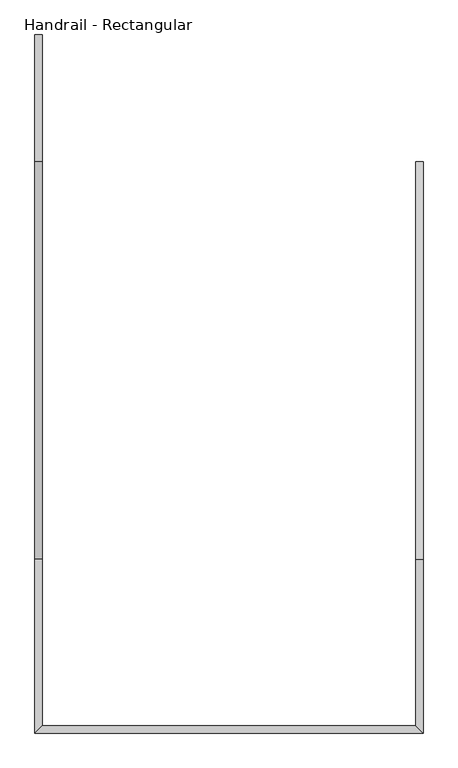
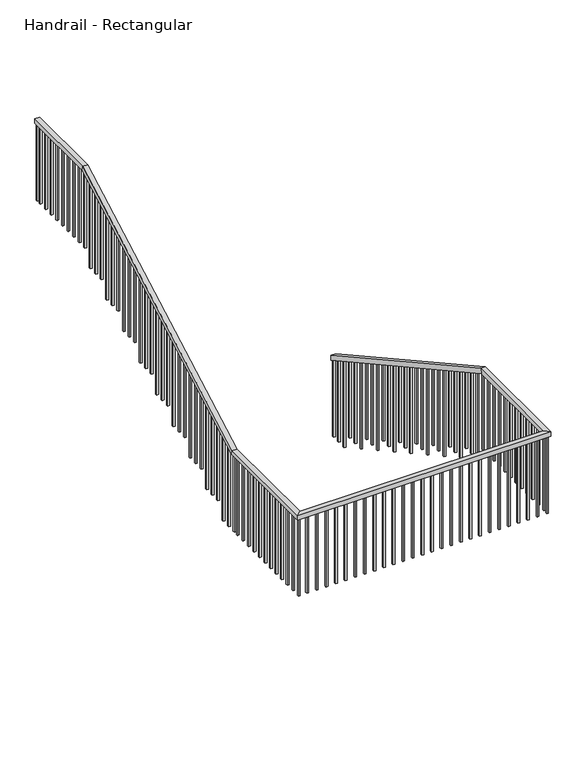
"""IFC4 building model written with IfcOpenShell, lengths in millimetres: railing geometry, Handrail - Rectangular."""

from ifc_helpers import new_model, si_unit, frame, origin, place, context, project, spatial, polyline, outline, extrude, faceted_brep, source, transform, mapped, element, save


def handrail_rectangular_0e0fe6d2(model_context):
    return source(origin(), model_context, "Body", "SolidModel", [
        faceted_brep([(-73320.227375, 12915.9, 10449.0921053), (-73269.427375, 12915.9, 10449.0921053), (-73269.427375, 12915.9, 10391.0509841), (-73320.227375, 12915.9, 10391.0509841), (-73320.227375, 10172.7, 11965.0710526), (-73269.427375, 10172.7, 11965.0710526), (-73269.427375, 10159.5970189, 11914.2710526), (-73320.227375, 10159.5970189, 11914.2710526), (-73320.227375, 9023.35, 11965.0710526), (-73269.427375, 8972.55, 11965.0710526), (-73269.427375, 8972.55, 11914.2710526), (-73320.227375, 9023.35, 11914.2710526), (-75898.327375, 9023.35, 11965.0710526), (-75949.127375, 8972.55, 11965.0710526), (-75949.127375, 8972.55, 11914.2710526), (-75898.327375, 9023.35, 11914.2710526), (-75898.327375, 10172.7, 11965.0710526), (-75949.127375, 10172.7, 11965.0710526), (-75949.127375, 10185.8029811, 11914.2710526), (-75898.327375, 10185.8029811, 11914.2710526), (-75898.327375, 12915.9, 13481.05), (-75949.127375, 12915.9, 13481.05), (-75949.127375, 12929.0029811, 13430.25), (-75898.327375, 12929.0029811, 13430.25), (-75898.327375, 13792.2, 13481.05), (-75898.327375, 13792.2, 13430.25), (-75949.127375, 13792.2, 13430.25), (-75949.127375, 13792.2, 13481.05)], [[[0, 1, 2, 3]], [[1, 0, 4, 5]], [[2, 1, 5, 6]], [[3, 2, 6, 7]], [[0, 3, 7, 4]], [[5, 4, 8, 9]], [[6, 5, 9, 10]], [[7, 6, 10, 11]], [[4, 7, 11, 8]], [[9, 8, 12, 13]], [[10, 9, 13, 14]], [[11, 10, 14, 15]], [[8, 11, 15, 12]], [[13, 12, 16, 17]], [[14, 13, 17, 18]], [[15, 14, 18, 19]], [[12, 15, 19, 16]], [[17, 16, 20, 21]], [[18, 17, 21, 22]], [[19, 18, 22, 23]], [[16, 19, 23, 20]], [[24, 25, 26, 27]], [[21, 20, 24, 27]], [[22, 21, 27, 26]], [[23, 22, 26, 25]], [[20, 23, 25, 24]]]),
        extrude(outline(polyline([(-75914.202375, 13719.175), (-75933.252375, 13719.175), (-75933.252375, 13738.225), (-75914.202375, 13738.225), (-75914.202375, 13719.175)])), frame((0.0, 0.0, 12566.65), z_axis=(0.0, 0.0, 1.0), x_axis=(1.0, 0.0, 0.0)), (0.0, 0.0, 1.0), 863.6),
        extrude(outline(polyline([(-75914.202375, 13617.575), (-75933.252375, 13617.575), (-75933.252375, 13636.625), (-75914.202375, 13636.625), (-75914.202375, 13617.575)])), frame((0.0, 0.0, 12566.65), z_axis=(0.0, 0.0, 1.0), x_axis=(1.0, 0.0, 0.0)), (0.0, 0.0, 1.0), 863.6),
        extrude(outline(polyline([(-75914.202375, 13515.975), (-75933.252375, 13515.975), (-75933.252375, 13535.025), (-75914.202375, 13535.025), (-75914.202375, 13515.975)])), frame((0.0, 0.0, 12566.65), z_axis=(0.0, 0.0, 1.0), x_axis=(1.0, 0.0, 0.0)), (0.0, 0.0, 1.0), 863.6),
        extrude(outline(polyline([(-75914.202375, 13414.375), (-75933.252375, 13414.375), (-75933.252375, 13433.425), (-75914.202375, 13433.425), (-75914.202375, 13414.375)])), frame((0.0, 0.0, 12566.65), z_axis=(0.0, 0.0, 1.0), x_axis=(1.0, 0.0, 0.0)), (0.0, 0.0, 1.0), 863.6),
        extrude(outline(polyline([(-75914.202375, 13312.775), (-75933.252375, 13312.775), (-75933.252375, 13331.825), (-75914.202375, 13331.825), (-75914.202375, 13312.775)])), frame((0.0, 0.0, 12566.65), z_axis=(0.0, 0.0, 1.0), x_axis=(1.0, 0.0, 0.0)), (0.0, 0.0, 1.0), 863.6),
        extrude(outline(polyline([(-75914.202375, 13211.175), (-75933.252375, 13211.175), (-75933.252375, 13230.225), (-75914.202375, 13230.225), (-75914.202375, 13211.175)])), frame((0.0, 0.0, 12566.65), z_axis=(0.0, 0.0, 1.0), x_axis=(1.0, 0.0, 0.0)), (0.0, 0.0, 1.0), 863.6),
        extrude(outline(polyline([(-75914.202375, 13109.575), (-75933.252375, 13109.575), (-75933.252375, 13128.625), (-75914.202375, 13128.625), (-75914.202375, 13109.575)])), frame((0.0, 0.0, 12566.65), z_axis=(0.0, 0.0, 1.0), x_axis=(1.0, 0.0, 0.0)), (0.0, 0.0, 1.0), 863.6),
        extrude(outline(polyline([(-75914.202375, 13007.975), (-75933.252375, 13007.975), (-75933.252375, 13027.025), (-75914.202375, 13027.025), (-75914.202375, 13007.975)])), frame((0.0, 0.0, 12566.65), z_axis=(0.0, 0.0, 1.0), x_axis=(1.0, 0.0, 0.0)), (0.0, 0.0, 1.0), 863.6),
        extrude(outline(polyline([(12804.775, 13361.5976946), (12823.825, 13372.1253262), (12823.825, 12398.2078947), (12804.775, 12398.2078947), (12804.775, 13361.5976946)])), frame((-75933.252375, 0.0, 0.0), z_axis=(1.0, 0.0, 0.0), x_axis=(0.0, 1.0, 0.0)), (0.0, 0.0, 1.0), 19.05),
        extrude(outline(polyline([(12703.175, 13305.4503262), (12722.225, 13315.9779578), (12722.225, 12398.2078947), (12703.175, 12398.2078947), (12703.175, 13305.4503262)])), frame((-75933.252375, 0.0, 0.0), z_axis=(1.0, 0.0, 0.0), x_axis=(0.0, 1.0, 0.0)), (0.0, 0.0, 1.0), 19.05),
        extrude(outline(polyline([(12601.575, 13249.3029578), (12620.625, 13259.8305894), (12620.625, 12398.2078947), (12601.575, 12398.2078947), (12601.575, 13249.3029578)])), frame((-75933.252375, 0.0, 0.0), z_axis=(1.0, 0.0, 0.0), x_axis=(0.0, 1.0, 0.0)), (0.0, 0.0, 1.0), 19.05),
        extrude(outline(polyline([(12499.975, 13193.1555894), (12519.025, 13203.6832209), (12519.025, 12229.7657895), (12499.975, 12229.7657895), (12499.975, 13193.1555894)])), frame((-75933.252375, 0.0, 0.0), z_axis=(1.0, 0.0, 0.0), x_axis=(0.0, 1.0, 0.0)), (0.0, 0.0, 1.0), 19.05),
        extrude(outline(polyline([(12398.375, 13137.0082209), (12417.425, 13147.5358525), (12417.425, 12229.7657895), (12398.375, 12229.7657895), (12398.375, 13137.0082209)])), frame((-75933.252375, 0.0, 0.0), z_axis=(1.0, 0.0, 0.0), x_axis=(0.0, 1.0, 0.0)), (0.0, 0.0, 1.0), 19.05),
        extrude(outline(polyline([(12296.775, 13080.8608525), (12315.825, 13091.3884841), (12315.825, 12229.7657895), (12296.775, 12229.7657895), (12296.775, 13080.8608525)])), frame((-75933.252375, 0.0, 0.0), z_axis=(1.0, 0.0, 0.0), x_axis=(0.0, 1.0, 0.0)), (0.0, 0.0, 1.0), 19.05),
        extrude(outline(polyline([(12195.175, 13024.7134841), (12214.225, 13035.2411157), (12214.225, 12061.3236842), (12195.175, 12061.3236842), (12195.175, 13024.7134841)])), frame((-75933.252375, 0.0, 0.0), z_axis=(1.0, 0.0, 0.0), x_axis=(0.0, 1.0, 0.0)), (0.0, 0.0, 1.0), 19.05),
        extrude(outline(polyline([(12093.575, 12968.5661157), (12112.625, 12979.0937473), (12112.625, 12061.3236842), (12093.575, 12061.3236842), (12093.575, 12968.5661157)])), frame((-75933.252375, 0.0, 0.0), z_axis=(1.0, 0.0, 0.0), x_axis=(0.0, 1.0, 0.0)), (0.0, 0.0, 1.0), 19.05),
        extrude(outline(polyline([(11991.975, 12912.4187473), (12011.025, 12922.9463788), (12011.025, 12061.3236842), (11991.975, 12061.3236842), (11991.975, 12912.4187473)])), frame((-75933.252375, 0.0, 0.0), z_axis=(1.0, 0.0, 0.0), x_axis=(0.0, 1.0, 0.0)), (0.0, 0.0, 1.0), 19.05),
        extrude(outline(polyline([(11890.375, 12856.2713788), (11909.425, 12866.7990104), (11909.425, 11892.8815789), (11890.375, 11892.8815789), (11890.375, 12856.2713788)])), frame((-75933.252375, 0.0, 0.0), z_axis=(1.0, 0.0, 0.0), x_axis=(0.0, 1.0, 0.0)), (0.0, 0.0, 1.0), 19.05),
        extrude(outline(polyline([(11788.775, 12800.1240104), (11807.825, 12810.651642), (11807.825, 11892.8815789), (11788.775, 11892.8815789), (11788.775, 12800.1240104)])), frame((-75933.252375, 0.0, 0.0), z_axis=(1.0, 0.0, 0.0), x_axis=(0.0, 1.0, 0.0)), (0.0, 0.0, 1.0), 19.05),
        extrude(outline(polyline([(11687.175, 12743.976642), (11706.225, 12754.5042736), (11706.225, 11892.8815789), (11687.175, 11892.8815789), (11687.175, 12743.976642)])), frame((-75933.252375, 0.0, 0.0), z_axis=(1.0, 0.0, 0.0), x_axis=(0.0, 1.0, 0.0)), (0.0, 0.0, 1.0), 19.05),
        extrude(outline(polyline([(11585.575, 12687.8292736), (11604.625, 12698.3569052), (11604.625, 11724.4394737), (11585.575, 11724.4394737), (11585.575, 12687.8292736)])), frame((-75933.252375, 0.0, 0.0), z_axis=(1.0, 0.0, 0.0), x_axis=(0.0, 1.0, 0.0)), (0.0, 0.0, 1.0), 19.05),
        extrude(outline(polyline([(11483.975, 12631.6819052), (11503.025, 12642.2095367), (11503.025, 11724.4394737), (11483.975, 11724.4394737), (11483.975, 12631.6819052)])), frame((-75933.252375, 0.0, 0.0), z_axis=(1.0, 0.0, 0.0), x_axis=(0.0, 1.0, 0.0)), (0.0, 0.0, 1.0), 19.05),
        extrude(outline(polyline([(11382.375, 12575.5345367), (11401.425, 12586.0621683), (11401.425, 11724.4394737), (11382.375, 11724.4394737), (11382.375, 12575.5345367)])), frame((-75933.252375, 0.0, 0.0), z_axis=(1.0, 0.0, 0.0), x_axis=(0.0, 1.0, 0.0)), (0.0, 0.0, 1.0), 19.05),
        extrude(outline(polyline([(11280.775, 12519.3871683), (11299.825, 12529.9147999), (11299.825, 11555.9973684), (11280.775, 11555.9973684), (11280.775, 12519.3871683)])), frame((-75933.252375, 0.0, 0.0), z_axis=(1.0, 0.0, 0.0), x_axis=(0.0, 1.0, 0.0)), (0.0, 0.0, 1.0), 19.05),
        extrude(outline(polyline([(11179.175, 12463.2397999), (11198.225, 12473.7674315), (11198.225, 11555.9973684), (11179.175, 11555.9973684), (11179.175, 12463.2397999)])), frame((-75933.252375, 0.0, 0.0), z_axis=(1.0, 0.0, 0.0), x_axis=(0.0, 1.0, 0.0)), (0.0, 0.0, 1.0), 19.05),
        extrude(outline(polyline([(11077.575, 12407.0924315), (11096.625, 12417.6200631), (11096.625, 11555.9973684), (11077.575, 11555.9973684), (11077.575, 12407.0924315)])), frame((-75933.252375, 0.0, 0.0), z_axis=(1.0, 0.0, 0.0), x_axis=(0.0, 1.0, 0.0)), (0.0, 0.0, 1.0), 19.05),
        extrude(outline(polyline([(10975.975, 12350.9450631), (10995.025, 12361.4726946), (10995.025, 11387.5552632), (10975.975, 11387.5552632), (10975.975, 12350.9450631)])), frame((-75933.252375, 0.0, 0.0), z_axis=(1.0, 0.0, 0.0), x_axis=(0.0, 1.0, 0.0)), (0.0, 0.0, 1.0), 19.05),
        extrude(outline(polyline([(10874.375, 12294.7976946), (10893.425, 12305.3253262), (10893.425, 11387.5552632), (10874.375, 11387.5552632), (10874.375, 12294.7976946)])), frame((-75933.252375, 0.0, 0.0), z_axis=(1.0, 0.0, 0.0), x_axis=(0.0, 1.0, 0.0)), (0.0, 0.0, 1.0), 19.05),
        extrude(outline(polyline([(10772.775, 12238.6503262), (10791.825, 12249.1779578), (10791.825, 11387.5552632), (10772.775, 11387.5552632), (10772.775, 12238.6503262)])), frame((-75933.252375, 0.0, 0.0), z_axis=(1.0, 0.0, 0.0), x_axis=(0.0, 1.0, 0.0)), (0.0, 0.0, 1.0), 19.05),
        extrude(outline(polyline([(10671.175, 12182.5029578), (10690.225, 12193.0305894), (10690.225, 11219.1131579), (10671.175, 11219.1131579), (10671.175, 12182.5029578)])), frame((-75933.252375, 0.0, 0.0), z_axis=(1.0, 0.0, 0.0), x_axis=(0.0, 1.0, 0.0)), (0.0, 0.0, 1.0), 19.05),
        extrude(outline(polyline([(10569.575, 12126.3555894), (10588.625, 12136.8832209), (10588.625, 11219.1131579), (10569.575, 11219.1131579), (10569.575, 12126.3555894)])), frame((-75933.252375, 0.0, 0.0), z_axis=(1.0, 0.0, 0.0), x_axis=(0.0, 1.0, 0.0)), (0.0, 0.0, 1.0), 19.05),
        extrude(outline(polyline([(10467.975, 12070.2082209), (10487.025, 12080.7358525), (10487.025, 11219.1131579), (10467.975, 11219.1131579), (10467.975, 12070.2082209)])), frame((-75933.252375, 0.0, 0.0), z_axis=(1.0, 0.0, 0.0), x_axis=(0.0, 1.0, 0.0)), (0.0, 0.0, 1.0), 19.05),
        extrude(outline(polyline([(10366.375, 12014.0608525), (10385.425, 12024.5884841), (10385.425, 11050.6710526), (10366.375, 11050.6710526), (10366.375, 12014.0608525)])), frame((-75933.252375, 0.0, 0.0), z_axis=(1.0, 0.0, 0.0), x_axis=(0.0, 1.0, 0.0)), (0.0, 0.0, 1.0), 19.05),
        extrude(outline(polyline([(10264.775, 11957.9134841), (10283.825, 11968.4411157), (10283.825, 11050.6710526), (10264.775, 11050.6710526), (10264.775, 11957.9134841)])), frame((-75933.252375, 0.0, 0.0), z_axis=(1.0, 0.0, 0.0), x_axis=(0.0, 1.0, 0.0)), (0.0, 0.0, 1.0), 19.05),
        extrude(outline(polyline([(-75914.202375, 10106.025), (-75933.252375, 10106.025), (-75933.252375, 10125.075), (-75914.202375, 10125.075), (-75914.202375, 10106.025)])), frame((0.0, 0.0, 11050.6710526), z_axis=(0.0, 0.0, 1.0), x_axis=(1.0, 0.0, 0.0)), (0.0, 0.0, 1.0), 863.6),
        extrude(outline(polyline([(-75914.202375, 10004.425), (-75933.252375, 10004.425), (-75933.252375, 10023.475), (-75914.202375, 10023.475), (-75914.202375, 10004.425)])), frame((0.0, 0.0, 11050.6710526), z_axis=(0.0, 0.0, 1.0), x_axis=(1.0, 0.0, 0.0)), (0.0, 0.0, 1.0), 863.6),
        extrude(outline(polyline([(-75914.202375, 9902.825), (-75933.252375, 9902.825), (-75933.252375, 9921.875), (-75914.202375, 9921.875), (-75914.202375, 9902.825)])), frame((0.0, 0.0, 11050.6710526), z_axis=(0.0, 0.0, 1.0), x_axis=(1.0, 0.0, 0.0)), (0.0, 0.0, 1.0), 863.6),
        extrude(outline(polyline([(-75914.202375, 9801.225), (-75933.252375, 9801.225), (-75933.252375, 9820.275), (-75914.202375, 9820.275), (-75914.202375, 9801.225)])), frame((0.0, 0.0, 11050.6710526), z_axis=(0.0, 0.0, 1.0), x_axis=(1.0, 0.0, 0.0)), (0.0, 0.0, 1.0), 863.6),
        extrude(outline(polyline([(-75914.202375, 9699.625), (-75933.252375, 9699.625), (-75933.252375, 9718.675), (-75914.202375, 9718.675), (-75914.202375, 9699.625)])), frame((0.0, 0.0, 11050.6710526), z_axis=(0.0, 0.0, 1.0), x_axis=(1.0, 0.0, 0.0)), (0.0, 0.0, 1.0), 863.6),
        extrude(outline(polyline([(-75914.202375, 9598.025), (-75933.252375, 9598.025), (-75933.252375, 9617.075), (-75914.202375, 9617.075), (-75914.202375, 9598.025)])), frame((0.0, 0.0, 11050.6710526), z_axis=(0.0, 0.0, 1.0), x_axis=(1.0, 0.0, 0.0)), (0.0, 0.0, 1.0), 863.6),
        extrude(outline(polyline([(-75914.202375, 9496.425), (-75933.252375, 9496.425), (-75933.252375, 9515.475), (-75914.202375, 9515.475), (-75914.202375, 9496.425)])), frame((0.0, 0.0, 11050.6710526), z_axis=(0.0, 0.0, 1.0), x_axis=(1.0, 0.0, 0.0)), (0.0, 0.0, 1.0), 863.6),
        extrude(outline(polyline([(-75914.202375, 9394.825), (-75933.252375, 9394.825), (-75933.252375, 9413.875), (-75914.202375, 9413.875), (-75914.202375, 9394.825)])), frame((0.0, 0.0, 11050.6710526), z_axis=(0.0, 0.0, 1.0), x_axis=(1.0, 0.0, 0.0)), (0.0, 0.0, 1.0), 863.6),
        extrude(outline(polyline([(-75914.202375, 9293.225), (-75933.252375, 9293.225), (-75933.252375, 9312.275), (-75914.202375, 9312.275), (-75914.202375, 9293.225)])), frame((0.0, 0.0, 11050.6710526), z_axis=(0.0, 0.0, 1.0), x_axis=(1.0, 0.0, 0.0)), (0.0, 0.0, 1.0), 863.6),
        extrude(outline(polyline([(-75914.202375, 9191.625), (-75933.252375, 9191.625), (-75933.252375, 9210.675), (-75914.202375, 9210.675), (-75914.202375, 9191.625)])), frame((0.0, 0.0, 11050.6710526), z_axis=(0.0, 0.0, 1.0), x_axis=(1.0, 0.0, 0.0)), (0.0, 0.0, 1.0), 863.6),
        extrude(outline(polyline([(-75914.202375, 9090.025), (-75933.252375, 9090.025), (-75933.252375, 9109.075), (-75914.202375, 9109.075), (-75914.202375, 9090.025)])), frame((0.0, 0.0, 11050.6710526), z_axis=(0.0, 0.0, 1.0), x_axis=(1.0, 0.0, 0.0)), (0.0, 0.0, 1.0), 863.6),
        extrude(outline(polyline([(-75825.302375, 9007.475), (-75825.302375, 8988.425), (-75844.352375, 8988.425), (-75844.352375, 9007.475), (-75825.302375, 9007.475)])), frame((0.0, 0.0, 11050.6710526), z_axis=(0.0, 0.0, 1.0), x_axis=(1.0, 0.0, 0.0)), (0.0, 0.0, 1.0), 863.6),
        extrude(outline(polyline([(-75723.702375, 9007.475), (-75723.702375, 8988.425), (-75742.752375, 8988.425), (-75742.752375, 9007.475), (-75723.702375, 9007.475)])), frame((0.0, 0.0, 11050.6710526), z_axis=(0.0, 0.0, 1.0), x_axis=(1.0, 0.0, 0.0)), (0.0, 0.0, 1.0), 863.6),
        extrude(outline(polyline([(-75622.102375, 9007.475), (-75622.102375, 8988.425), (-75641.152375, 8988.425), (-75641.152375, 9007.475), (-75622.102375, 9007.475)])), frame((0.0, 0.0, 11050.6710526), z_axis=(0.0, 0.0, 1.0), x_axis=(1.0, 0.0, 0.0)), (0.0, 0.0, 1.0), 863.6),
        extrude(outline(polyline([(-75520.502375, 9007.475), (-75520.502375, 8988.425), (-75539.552375, 8988.425), (-75539.552375, 9007.475), (-75520.502375, 9007.475)])), frame((0.0, 0.0, 11050.6710526), z_axis=(0.0, 0.0, 1.0), x_axis=(1.0, 0.0, 0.0)), (0.0, 0.0, 1.0), 863.6),
        extrude(outline(polyline([(-75418.902375, 9007.475), (-75418.902375, 8988.425), (-75437.952375, 8988.425), (-75437.952375, 9007.475), (-75418.902375, 9007.475)])), frame((0.0, 0.0, 11050.6710526), z_axis=(0.0, 0.0, 1.0), x_axis=(1.0, 0.0, 0.0)), (0.0, 0.0, 1.0), 863.6),
        extrude(outline(polyline([(-75317.302375, 9007.475), (-75317.302375, 8988.425), (-75336.352375, 8988.425), (-75336.352375, 9007.475), (-75317.302375, 9007.475)])), frame((0.0, 0.0, 11050.6710526), z_axis=(0.0, 0.0, 1.0), x_axis=(1.0, 0.0, 0.0)), (0.0, 0.0, 1.0), 863.6),
        extrude(outline(polyline([(-75215.702375, 9007.475), (-75215.702375, 8988.425), (-75234.752375, 8988.425), (-75234.752375, 9007.475), (-75215.702375, 9007.475)])), frame((0.0, 0.0, 11050.6710526), z_axis=(0.0, 0.0, 1.0), x_axis=(1.0, 0.0, 0.0)), (0.0, 0.0, 1.0), 863.6),
        extrude(outline(polyline([(-75114.102375, 9007.475), (-75114.102375, 8988.425), (-75133.152375, 8988.425), (-75133.152375, 9007.475), (-75114.102375, 9007.475)])), frame((0.0, 0.0, 11050.6710526), z_axis=(0.0, 0.0, 1.0), x_axis=(1.0, 0.0, 0.0)), (0.0, 0.0, 1.0), 863.6),
        extrude(outline(polyline([(-75012.502375, 9007.475), (-75012.502375, 8988.425), (-75031.552375, 8988.425), (-75031.552375, 9007.475), (-75012.502375, 9007.475)])), frame((0.0, 0.0, 11050.6710526), z_axis=(0.0, 0.0, 1.0), x_axis=(1.0, 0.0, 0.0)), (0.0, 0.0, 1.0), 863.6),
        extrude(outline(polyline([(-74910.902375, 9007.475), (-74910.902375, 8988.425), (-74929.952375, 8988.425), (-74929.952375, 9007.475), (-74910.902375, 9007.475)])), frame((0.0, 0.0, 11050.6710526), z_axis=(0.0, 0.0, 1.0), x_axis=(1.0, 0.0, 0.0)), (0.0, 0.0, 1.0), 863.6),
        extrude(outline(polyline([(-74809.302375, 9007.475), (-74809.302375, 8988.425), (-74828.352375, 8988.425), (-74828.352375, 9007.475), (-74809.302375, 9007.475)])), frame((0.0, 0.0, 11050.6710526), z_axis=(0.0, 0.0, 1.0), x_axis=(1.0, 0.0, 0.0)), (0.0, 0.0, 1.0), 863.6),
        extrude(outline(polyline([(-74707.702375, 9007.475), (-74707.702375, 8988.425), (-74726.752375, 8988.425), (-74726.752375, 9007.475), (-74707.702375, 9007.475)])), frame((0.0, 0.0, 11050.6710526), z_axis=(0.0, 0.0, 1.0), x_axis=(1.0, 0.0, 0.0)), (0.0, 0.0, 1.0), 863.6),
        extrude(outline(polyline([(-74606.102375, 9007.475), (-74606.102375, 8988.425), (-74625.152375, 8988.425), (-74625.152375, 9007.475), (-74606.102375, 9007.475)])), frame((0.0, 0.0, 11050.6710526), z_axis=(0.0, 0.0, 1.0), x_axis=(1.0, 0.0, 0.0)), (0.0, 0.0, 1.0), 863.6),
        extrude(outline(polyline([(-74504.502375, 9007.475), (-74504.502375, 8988.425), (-74523.552375, 8988.425), (-74523.552375, 9007.475), (-74504.502375, 9007.475)])), frame((0.0, 0.0, 11050.6710526), z_axis=(0.0, 0.0, 1.0), x_axis=(1.0, 0.0, 0.0)), (0.0, 0.0, 1.0), 863.6),
        extrude(outline(polyline([(-74402.902375, 9007.475), (-74402.902375, 8988.425), (-74421.952375, 8988.425), (-74421.952375, 9007.475), (-74402.902375, 9007.475)])), frame((0.0, 0.0, 11050.6710526), z_axis=(0.0, 0.0, 1.0), x_axis=(1.0, 0.0, 0.0)), (0.0, 0.0, 1.0), 863.6),
        extrude(outline(polyline([(-74301.302375, 9007.475), (-74301.302375, 8988.425), (-74320.352375, 8988.425), (-74320.352375, 9007.475), (-74301.302375, 9007.475)])), frame((0.0, 0.0, 11050.6710526), z_axis=(0.0, 0.0, 1.0), x_axis=(1.0, 0.0, 0.0)), (0.0, 0.0, 1.0), 863.6),
        extrude(outline(polyline([(-74199.702375, 9007.475), (-74199.702375, 8988.425), (-74218.752375, 8988.425), (-74218.752375, 9007.475), (-74199.702375, 9007.475)])), frame((0.0, 0.0, 11050.6710526), z_axis=(0.0, 0.0, 1.0), x_axis=(1.0, 0.0, 0.0)), (0.0, 0.0, 1.0), 863.6),
        extrude(outline(polyline([(-74098.102375, 9007.475), (-74098.102375, 8988.425), (-74117.152375, 8988.425), (-74117.152375, 9007.475), (-74098.102375, 9007.475)])), frame((0.0, 0.0, 11050.6710526), z_axis=(0.0, 0.0, 1.0), x_axis=(1.0, 0.0, 0.0)), (0.0, 0.0, 1.0), 863.6),
        extrude(outline(polyline([(-73996.502375, 9007.475), (-73996.502375, 8988.425), (-74015.552375, 8988.425), (-74015.552375, 9007.475), (-73996.502375, 9007.475)])), frame((0.0, 0.0, 11050.6710526), z_axis=(0.0, 0.0, 1.0), x_axis=(1.0, 0.0, 0.0)), (0.0, 0.0, 1.0), 863.6),
        extrude(outline(polyline([(-73894.902375, 9007.475), (-73894.902375, 8988.425), (-73913.952375, 8988.425), (-73913.952375, 9007.475), (-73894.902375, 9007.475)])), frame((0.0, 0.0, 11050.6710526), z_axis=(0.0, 0.0, 1.0), x_axis=(1.0, 0.0, 0.0)), (0.0, 0.0, 1.0), 863.6),
        extrude(outline(polyline([(-73793.302375, 9007.475), (-73793.302375, 8988.425), (-73812.352375, 8988.425), (-73812.352375, 9007.475), (-73793.302375, 9007.475)])), frame((0.0, 0.0, 11050.6710526), z_axis=(0.0, 0.0, 1.0), x_axis=(1.0, 0.0, 0.0)), (0.0, 0.0, 1.0), 863.6),
        extrude(outline(polyline([(-73691.702375, 9007.475), (-73691.702375, 8988.425), (-73710.752375, 8988.425), (-73710.752375, 9007.475), (-73691.702375, 9007.475)])), frame((0.0, 0.0, 11050.6710526), z_axis=(0.0, 0.0, 1.0), x_axis=(1.0, 0.0, 0.0)), (0.0, 0.0, 1.0), 863.6),
        extrude(outline(polyline([(-73590.102375, 9007.475), (-73590.102375, 8988.425), (-73609.152375, 8988.425), (-73609.152375, 9007.475), (-73590.102375, 9007.475)])), frame((0.0, 0.0, 11050.6710526), z_axis=(0.0, 0.0, 1.0), x_axis=(1.0, 0.0, 0.0)), (0.0, 0.0, 1.0), 863.6),
        extrude(outline(polyline([(-73488.502375, 9007.475), (-73488.502375, 8988.425), (-73507.552375, 8988.425), (-73507.552375, 9007.475), (-73488.502375, 9007.475)])), frame((0.0, 0.0, 11050.6710526), z_axis=(0.0, 0.0, 1.0), x_axis=(1.0, 0.0, 0.0)), (0.0, 0.0, 1.0), 863.6),
        extrude(outline(polyline([(-73386.902375, 9007.475), (-73386.902375, 8988.425), (-73405.952375, 8988.425), (-73405.952375, 9007.475), (-73386.902375, 9007.475)])), frame((0.0, 0.0, 11050.6710526), z_axis=(0.0, 0.0, 1.0), x_axis=(1.0, 0.0, 0.0)), (0.0, 0.0, 1.0), 863.6),
        extrude(outline(polyline([(-73304.352375, 9064.625), (-73285.302375, 9064.625), (-73285.302375, 9045.575), (-73304.352375, 9045.575), (-73304.352375, 9064.625)])), frame((0.0, 0.0, 11050.6710526), z_axis=(0.0, 0.0, 1.0), x_axis=(1.0, 0.0, 0.0)), (0.0, 0.0, 1.0), 863.6),
        extrude(outline(polyline([(-73304.352375, 9166.225), (-73285.302375, 9166.225), (-73285.302375, 9147.175), (-73304.352375, 9147.175), (-73304.352375, 9166.225)])), frame((0.0, 0.0, 11050.6710526), z_axis=(0.0, 0.0, 1.0), x_axis=(1.0, 0.0, 0.0)), (0.0, 0.0, 1.0), 863.6),
        extrude(outline(polyline([(-73304.352375, 9267.825), (-73285.302375, 9267.825), (-73285.302375, 9248.775), (-73304.352375, 9248.775), (-73304.352375, 9267.825)])), frame((0.0, 0.0, 11050.6710526), z_axis=(0.0, 0.0, 1.0), x_axis=(1.0, 0.0, 0.0)), (0.0, 0.0, 1.0), 863.6),
        extrude(outline(polyline([(-73304.352375, 9369.425), (-73285.302375, 9369.425), (-73285.302375, 9350.375), (-73304.352375, 9350.375), (-73304.352375, 9369.425)])), frame((0.0, 0.0, 11050.6710526), z_axis=(0.0, 0.0, 1.0), x_axis=(1.0, 0.0, 0.0)), (0.0, 0.0, 1.0), 863.6),
        extrude(outline(polyline([(-73304.352375, 9471.025), (-73285.302375, 9471.025), (-73285.302375, 9451.975), (-73304.352375, 9451.975), (-73304.352375, 9471.025)])), frame((0.0, 0.0, 11050.6710526), z_axis=(0.0, 0.0, 1.0), x_axis=(1.0, 0.0, 0.0)), (0.0, 0.0, 1.0), 863.6),
        extrude(outline(polyline([(-73304.352375, 9572.625), (-73285.302375, 9572.625), (-73285.302375, 9553.575), (-73304.352375, 9553.575), (-73304.352375, 9572.625)])), frame((0.0, 0.0, 11050.6710526), z_axis=(0.0, 0.0, 1.0), x_axis=(1.0, 0.0, 0.0)), (0.0, 0.0, 1.0), 863.6),
        extrude(outline(polyline([(-73304.352375, 9674.225), (-73285.302375, 9674.225), (-73285.302375, 9655.175), (-73304.352375, 9655.175), (-73304.352375, 9674.225)])), frame((0.0, 0.0, 11050.6710526), z_axis=(0.0, 0.0, 1.0), x_axis=(1.0, 0.0, 0.0)), (0.0, 0.0, 1.0), 863.6),
        extrude(outline(polyline([(-73304.352375, 9775.825), (-73285.302375, 9775.825), (-73285.302375, 9756.775), (-73304.352375, 9756.775), (-73304.352375, 9775.825)])), frame((0.0, 0.0, 11050.6710526), z_axis=(0.0, 0.0, 1.0), x_axis=(1.0, 0.0, 0.0)), (0.0, 0.0, 1.0), 863.6),
        extrude(outline(polyline([(-73304.352375, 9877.425), (-73285.302375, 9877.425), (-73285.302375, 9858.375), (-73304.352375, 9858.375), (-73304.352375, 9877.425)])), frame((0.0, 0.0, 11050.6710526), z_axis=(0.0, 0.0, 1.0), x_axis=(1.0, 0.0, 0.0)), (0.0, 0.0, 1.0), 863.6),
        extrude(outline(polyline([(-73304.352375, 9979.025), (-73285.302375, 9979.025), (-73285.302375, 9959.975), (-73304.352375, 9959.975), (-73304.352375, 9979.025)])), frame((0.0, 0.0, 11050.6710526), z_axis=(0.0, 0.0, 1.0), x_axis=(1.0, 0.0, 0.0)), (0.0, 0.0, 1.0), 863.6),
        extrude(outline(polyline([(-73304.352375, 10080.625), (-73285.302375, 10080.625), (-73285.302375, 10061.575), (-73304.352375, 10061.575), (-73304.352375, 10080.625)])), frame((0.0, 0.0, 11050.6710526), z_axis=(0.0, 0.0, 1.0), x_axis=(1.0, 0.0, 0.0)), (0.0, 0.0, 1.0), 863.6),
        extrude(outline(polyline([(10264.775, 11856.1463788), (10283.825, 11845.6187473), (10283.825, 10882.2289474), (10264.775, 10882.2289474), (10264.775, 11856.1463788)])), frame((-73304.352375, 0.0, 0.0), z_axis=(1.0, 0.0, 0.0), x_axis=(0.0, 1.0, 0.0)), (0.0, 0.0, 1.0), 19.05),
        extrude(outline(polyline([(10366.375, 11799.9990104), (10385.425, 11789.4713788), (10385.425, 10882.2289474), (10366.375, 10882.2289474), (10366.375, 11799.9990104)])), frame((-73304.352375, 0.0, 0.0), z_axis=(1.0, 0.0, 0.0), x_axis=(0.0, 1.0, 0.0)), (0.0, 0.0, 1.0), 19.05),
        extrude(outline(polyline([(10467.975, 11743.851642), (10487.025, 11733.3240104), (10487.025, 10882.2289474), (10467.975, 10882.2289474), (10467.975, 11743.851642)])), frame((-73304.352375, 0.0, 0.0), z_axis=(1.0, 0.0, 0.0), x_axis=(0.0, 1.0, 0.0)), (0.0, 0.0, 1.0), 19.05),
        extrude(outline(polyline([(10569.575, 11687.7042736), (10588.625, 11677.176642), (10588.625, 10713.7868421), (10569.575, 10713.7868421), (10569.575, 11687.7042736)])), frame((-73304.352375, 0.0, 0.0), z_axis=(1.0, 0.0, 0.0), x_axis=(0.0, 1.0, 0.0)), (0.0, 0.0, 1.0), 19.05),
        extrude(outline(polyline([(10671.175, 11631.5569052), (10690.225, 11621.0292736), (10690.225, 10713.7868421), (10671.175, 10713.7868421), (10671.175, 11631.5569052)])), frame((-73304.352375, 0.0, 0.0), z_axis=(1.0, 0.0, 0.0), x_axis=(0.0, 1.0, 0.0)), (0.0, 0.0, 1.0), 19.05),
        extrude(outline(polyline([(10772.775, 11575.4095367), (10791.825, 11564.8819052), (10791.825, 10713.7868421), (10772.775, 10713.7868421), (10772.775, 11575.4095367)])), frame((-73304.352375, 0.0, 0.0), z_axis=(1.0, 0.0, 0.0), x_axis=(0.0, 1.0, 0.0)), (0.0, 0.0, 1.0), 19.05),
        extrude(outline(polyline([(10874.375, 11519.2621683), (10893.425, 11508.7345367), (10893.425, 10545.3447368), (10874.375, 10545.3447368), (10874.375, 11519.2621683)])), frame((-73304.352375, 0.0, 0.0), z_axis=(1.0, 0.0, 0.0), x_axis=(0.0, 1.0, 0.0)), (0.0, 0.0, 1.0), 19.05),
        extrude(outline(polyline([(10975.975, 11463.1147999), (10995.025, 11452.5871683), (10995.025, 10545.3447368), (10975.975, 10545.3447368), (10975.975, 11463.1147999)])), frame((-73304.352375, 0.0, 0.0), z_axis=(1.0, 0.0, 0.0), x_axis=(0.0, 1.0, 0.0)), (0.0, 0.0, 1.0), 19.05),
        extrude(outline(polyline([(11077.575, 11406.9674315), (11096.625, 11396.4397999), (11096.625, 10545.3447368), (11077.575, 10545.3447368), (11077.575, 11406.9674315)])), frame((-73304.352375, 0.0, 0.0), z_axis=(1.0, 0.0, 0.0), x_axis=(0.0, 1.0, 0.0)), (0.0, 0.0, 1.0), 19.05),
        extrude(outline(polyline([(11179.175, 11350.8200631), (11198.225, 11340.2924315), (11198.225, 10376.9026316), (11179.175, 10376.9026316), (11179.175, 11350.8200631)])), frame((-73304.352375, 0.0, 0.0), z_axis=(1.0, 0.0, 0.0), x_axis=(0.0, 1.0, 0.0)), (0.0, 0.0, 1.0), 19.05),
        extrude(outline(polyline([(11280.775, 11294.6726946), (11299.825, 11284.1450631), (11299.825, 10376.9026316), (11280.775, 10376.9026316), (11280.775, 11294.6726946)])), frame((-73304.352375, 0.0, 0.0), z_axis=(1.0, 0.0, 0.0), x_axis=(0.0, 1.0, 0.0)), (0.0, 0.0, 1.0), 19.05),
        extrude(outline(polyline([(11382.375, 11238.5253262), (11401.425, 11227.9976946), (11401.425, 10376.9026316), (11382.375, 10376.9026316), (11382.375, 11238.5253262)])), frame((-73304.352375, 0.0, 0.0), z_axis=(1.0, 0.0, 0.0), x_axis=(0.0, 1.0, 0.0)), (0.0, 0.0, 1.0), 19.05),
        extrude(outline(polyline([(11483.975, 11182.3779578), (11503.025, 11171.8503262), (11503.025, 10208.4605263), (11483.975, 10208.4605263), (11483.975, 11182.3779578)])), frame((-73304.352375, 0.0, 0.0), z_axis=(1.0, 0.0, 0.0), x_axis=(0.0, 1.0, 0.0)), (0.0, 0.0, 1.0), 19.05),
        extrude(outline(polyline([(11585.575, 11126.2305894), (11604.625, 11115.7029578), (11604.625, 10208.4605263), (11585.575, 10208.4605263), (11585.575, 11126.2305894)])), frame((-73304.352375, 0.0, 0.0), z_axis=(1.0, 0.0, 0.0), x_axis=(0.0, 1.0, 0.0)), (0.0, 0.0, 1.0), 19.05),
        extrude(outline(polyline([(11687.175, 11070.0832209), (11706.225, 11059.5555894), (11706.225, 10208.4605263), (11687.175, 10208.4605263), (11687.175, 11070.0832209)])), frame((-73304.352375, 0.0, 0.0), z_axis=(1.0, 0.0, 0.0), x_axis=(0.0, 1.0, 0.0)), (0.0, 0.0, 1.0), 19.05),
        extrude(outline(polyline([(11788.775, 11013.9358525), (11807.825, 11003.4082209), (11807.825, 10040.0184211), (11788.775, 10040.0184211), (11788.775, 11013.9358525)])), frame((-73304.352375, 0.0, 0.0), z_axis=(1.0, 0.0, 0.0), x_axis=(0.0, 1.0, 0.0)), (0.0, 0.0, 1.0), 19.05),
        extrude(outline(polyline([(11890.375, 10957.7884841), (11909.425, 10947.2608525), (11909.425, 10040.0184211), (11890.375, 10040.0184211), (11890.375, 10957.7884841)])), frame((-73304.352375, 0.0, 0.0), z_axis=(1.0, 0.0, 0.0), x_axis=(0.0, 1.0, 0.0)), (0.0, 0.0, 1.0), 19.05),
        extrude(outline(polyline([(11991.975, 10901.6411157), (12011.025, 10891.1134841), (12011.025, 10040.0184211), (11991.975, 10040.0184211), (11991.975, 10901.6411157)])), frame((-73304.352375, 0.0, 0.0), z_axis=(1.0, 0.0, 0.0), x_axis=(0.0, 1.0, 0.0)), (0.0, 0.0, 1.0), 19.05),
        extrude(outline(polyline([(12093.575, 10845.4937473), (12112.625, 10834.9661157), (12112.625, 9871.5763158), (12093.575, 9871.5763158), (12093.575, 10845.4937473)])), frame((-73304.352375, 0.0, 0.0), z_axis=(1.0, 0.0, 0.0), x_axis=(0.0, 1.0, 0.0)), (0.0, 0.0, 1.0), 19.05),
        extrude(outline(polyline([(12195.175, 10789.3463788), (12214.225, 10778.8187473), (12214.225, 9871.5763158), (12195.175, 9871.5763158), (12195.175, 10789.3463788)])), frame((-73304.352375, 0.0, 0.0), z_axis=(1.0, 0.0, 0.0), x_axis=(0.0, 1.0, 0.0)), (0.0, 0.0, 1.0), 19.05),
        extrude(outline(polyline([(12296.775, 10733.1990104), (12315.825, 10722.6713788), (12315.825, 9871.5763158), (12296.775, 9871.5763158), (12296.775, 10733.1990104)])), frame((-73304.352375, 0.0, 0.0), z_axis=(1.0, 0.0, 0.0), x_axis=(0.0, 1.0, 0.0)), (0.0, 0.0, 1.0), 19.05),
        extrude(outline(polyline([(12398.375, 10677.051642), (12417.425, 10666.5240104), (12417.425, 9703.1342105), (12398.375, 9703.1342105), (12398.375, 10677.051642)])), frame((-73304.352375, 0.0, 0.0), z_axis=(1.0, 0.0, 0.0), x_axis=(0.0, 1.0, 0.0)), (0.0, 0.0, 1.0), 19.05),
        extrude(outline(polyline([(12499.975, 10620.9042736), (12519.025, 10610.376642), (12519.025, 9703.1342105), (12499.975, 9703.1342105), (12499.975, 10620.9042736)])), frame((-73304.352375, 0.0, 0.0), z_axis=(1.0, 0.0, 0.0), x_axis=(0.0, 1.0, 0.0)), (0.0, 0.0, 1.0), 19.05),
        extrude(outline(polyline([(12601.575, 10564.7569052), (12620.625, 10554.2292736), (12620.625, 9703.1342105), (12601.575, 9703.1342105), (12601.575, 10564.7569052)])), frame((-73304.352375, 0.0, 0.0), z_axis=(1.0, 0.0, 0.0), x_axis=(0.0, 1.0, 0.0)), (0.0, 0.0, 1.0), 19.05),
        extrude(outline(polyline([(12703.175, 10508.6095367), (12722.225, 10498.0819052), (12722.225, 9534.6921053), (12703.175, 9534.6921053), (12703.175, 10508.6095367)])), frame((-73304.352375, 0.0, 0.0), z_axis=(1.0, 0.0, 0.0), x_axis=(0.0, 1.0, 0.0)), (0.0, 0.0, 1.0), 19.05),
        extrude(outline(polyline([(12804.775, 10452.4621683), (12823.825, 10441.9345367), (12823.825, 9534.6921053), (12804.775, 9534.6921053), (12804.775, 10452.4621683)])), frame((-73304.352375, 0.0, 0.0), z_axis=(1.0, 0.0, 0.0), x_axis=(0.0, 1.0, 0.0)), (0.0, 0.0, 1.0), 19.05),
        extrude(outline(polyline([(12906.375, 13417.7450631), (12925.425, 13428.2726946), (12925.425, 12566.65), (12906.375, 12566.65), (12906.375, 13417.7450631)])), frame((-75933.252375, 0.0, 0.0), z_axis=(1.0, 0.0, 0.0), x_axis=(0.0, 1.0, 0.0)), (0.0, 0.0, 1.0), 19.05),
        extrude(outline(polyline([(-75914.202375, 10163.175), (-75933.252375, 10163.175), (-75933.252375, 10182.225), (-75914.202375, 10182.225), (-75914.202375, 10163.175)])), frame((0.0, 0.0, 11050.6710526), z_axis=(0.0, 0.0, 1.0), x_axis=(1.0, 0.0, 0.0)), (0.0, 0.0, 1.0), 863.6),
        extrude(outline(polyline([(-75914.202375, 9007.475), (-75914.202375, 8988.425), (-75933.252375, 8988.425), (-75933.252375, 9007.475), (-75914.202375, 9007.475)])), frame((0.0, 0.0, 11050.6710526), z_axis=(0.0, 0.0, 1.0), x_axis=(1.0, 0.0, 0.0)), (0.0, 0.0, 1.0), 863.6),
        extrude(outline(polyline([(-73304.352375, 9007.475), (-73285.302375, 9007.475), (-73285.302375, 8988.425), (-73304.352375, 8988.425), (-73304.352375, 9007.475)])), frame((0.0, 0.0, 11050.6710526), z_axis=(0.0, 0.0, 1.0), x_axis=(1.0, 0.0, 0.0)), (0.0, 0.0, 1.0), 863.6),
        extrude(outline(polyline([(10163.175, 11912.2937473), (10182.225, 11901.7661157), (10182.225, 11050.6710526), (10163.175, 11050.6710526), (10163.175, 11912.2937473)])), frame((-73304.352375, 0.0, 0.0), z_axis=(1.0, 0.0, 0.0), x_axis=(0.0, 1.0, 0.0)), (0.0, 0.0, 1.0), 19.05),
        extrude(outline(polyline([(-75914.202375, 13773.15), (-75933.252375, 13773.15), (-75933.252375, 13792.2), (-75914.202375, 13792.2), (-75914.202375, 13773.15)])), frame((0.0, 0.0, 12566.65), z_axis=(0.0, 0.0, 1.0), x_axis=(1.0, 0.0, 0.0)), (0.0, 0.0, 1.0), 863.6),
        extrude(outline(polyline([(12896.85, 10401.5786157), (12915.9, 10391.0509841), (12915.9, 9534.6921053), (12896.85, 9534.6921053), (12896.85, 10401.5786157)])), frame((-73304.352375, 0.0, 0.0), z_axis=(1.0, 0.0, 0.0), x_axis=(0.0, 1.0, 0.0)), (0.0, 0.0, 1.0), 19.05),
    ])


if __name__ == "__main__":
    model = new_model("IFC4")
    model_context = context("Model", 3, world=origin())
    ifc_project = project(units=[si_unit("LENGTHUNIT", "METRE", prefix="MILLI")], contexts=[model_context])
    site = spatial("IfcSite", under=ifc_project)
    building = spatial("IfcBuilding", under=site)
    placement = place(None, origin())
    handrail_rectangular_shape = handrail_rectangular_0e0fe6d2(model_context)
    element("IfcRailing", 1, ObjectType="Handrail - Rectangular", at=placement, inside=building, context=model_context, shape_type="MappedRepresentation", body=[
        mapped(handrail_rectangular_shape, transform((0.0, 0.0, 0.0), x_axis=(1.0, 0.0, 0.0), y_axis=(0.0, 1.0, 0.0), z_axis=(0.0, 0.0, 1.0))),
    ])
    save(model, "model.ifc")
